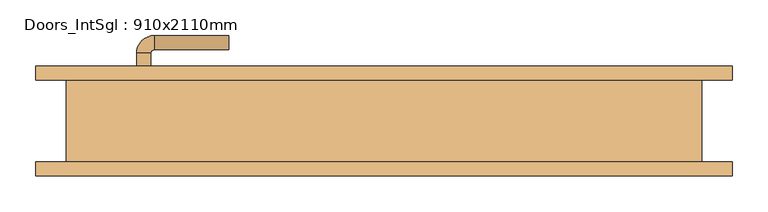
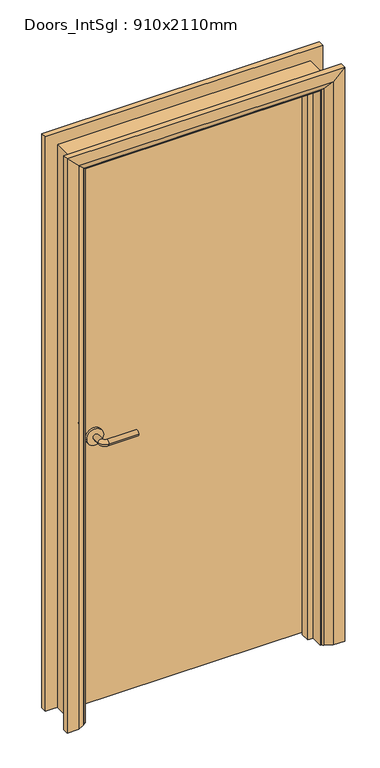
"""IFC4 building model written with IfcOpenShell, lengths in millimetres: door geometry, Doors_IntSgl : 910x2110mm."""

import ifcopenshell
import ifcopenshell.guid

model = None  # the IFC model being written
_history = None  # IfcOwnerHistory: only IFC2X3 demands one
_inside = {}  # id of a spatial element -> (the spatial element, [elements in it])
_under = {}  # id of a project, library or spatial element -> (it, [spatial elements below it])
_declared = {}  # id of a project -> (the project, [libraries it declares])
_typed = {}  # id of a type object -> (the type object, [elements of that type])
_made_of = {}  # id of a material, layer set ... -> (it, [elements and type objects made of it])


def new_model(schema):
    """Start an empty IFC model of exactly this schema.

    Asked for "IFC4X3", IfcOpenShell would pick the latest addendum, in which some entities
    have other attributes; the version numbers below select the first issue.
    IFC2X3 requires an IfcOwnerHistory on every rooted entity: one is made here for all.
    """
    global model, _history
    if schema == "IFC4X3":
        model = ifcopenshell.file(schema_version=(4, 3, 0, 0))
    else:
        model = ifcopenshell.file(schema=schema)
    _inside.clear()
    _under.clear()
    _declared.clear()
    _typed.clear()
    _made_of.clear()
    _history = None
    if model.schema == "IFC2X3":
        org = make("IfcOrganization", Name="unknown")
        user = make(
            "IfcPersonAndOrganization",
            ThePerson=make("IfcPerson", FamilyName="unknown"),
            TheOrganization=org,
        )
        app = make(
            "IfcApplication",
            ApplicationDeveloper=org,
            Version="unknown",
            ApplicationFullName="unknown",
            ApplicationIdentifier="unknown",
        )
        _history = make(
            "IfcOwnerHistory",
            OwningUser=user,
            OwningApplication=app,
            ChangeAction="ADDED",
            CreationDate=0,
        )
    return model


def make(cls, **values):
    """One entity of the class cls with the attributes given. An attribute that is None is left unset."""
    return model.create_entity(
        cls, **{name: value for name, value in values.items() if value is not None}
    )


def rooted(cls, **values):
    """An entity with a GlobalId (a new one), such as an element, a storey or a relation."""
    return make(cls, GlobalId=ifcopenshell.guid.new(), OwnerHistory=_history, **values)


def si_unit(unit_type, name, prefix=None):
    """IfcSIUnit, for example si_unit("LENGTHUNIT", "METRE", prefix="MILLI")."""
    return make("IfcSIUnit", UnitType=unit_type, Prefix=prefix, Name=name)


def assignment(units):
    """IfcUnitAssignment: the units of a project."""
    return None if units is None else make("IfcUnitAssignment", Units=units)


def point(xyz):
    """IfcCartesianPoint."""
    return None if xyz is None else make("IfcCartesianPoint", Coordinates=xyz)


def direction(xyz):
    """IfcDirection."""
    return None if xyz is None else make("IfcDirection", DirectionRatios=xyz)


def frame(location, z_axis=None, x_axis=None):
    """IfcAxis2Placement3D, a coordinate frame: its origin and axes. An axis left out is left unset."""
    return make(
        "IfcAxis2Placement3D",
        Location=point(location),
        Axis=direction(z_axis),
        RefDirection=direction(x_axis),
    )


def frame_2d(location, x_axis=None):
    """IfcAxis2Placement2D, a coordinate frame in the plane: its origin and x axis."""
    return make(
        "IfcAxis2Placement2D", Location=point(location), RefDirection=direction(x_axis)
    )


def origin():
    """The frame at (0, 0, 0) with its axes left unset."""
    return frame((0.0, 0.0, 0.0))


def place(relative_to, where):
    """IfcLocalPlacement: puts the frame where relative to a parent placement (None: the world)."""
    return make(
        "IfcLocalPlacement", PlacementRelTo=relative_to, RelativePlacement=where
    )


def context(
    kind, dimensions, precision=None, world=None, true_north=None, identifier=None
):
    """IfcGeometricRepresentationContext, for example the 3D "Model" context."""
    return make(
        "IfcGeometricRepresentationContext",
        ContextIdentifier=identifier,
        ContextType=kind,
        CoordinateSpaceDimension=dimensions,
        Precision=precision,
        WorldCoordinateSystem=world,
        TrueNorth=true_north,
    )


def project(units=None, contexts=None):
    """IfcProject with its units and contexts."""
    return rooted(
        "IfcProject",
        Name="project",
        RepresentationContexts=contexts,
        UnitsInContext=assignment(units),
    )


def spatial(cls, under=None, at=None, **own):
    """A site, building, storey or space (cls), placed at a placement, below another one or the project."""
    s = rooted(cls, ObjectPlacement=at, **own)
    if under is not None:
        _under.setdefault(under.id(), (under, []))[1].append(s)
    return s


def polyline(points):
    """IfcPolyline through the points."""
    return make("IfcPolyline", Points=[point(p) for p in points])


def circle_curve(where, radius):
    """IfcCircle in the frame where."""
    return make("IfcCircle", Position=where, Radius=radius)


def ellipse_curve(where, semi_axis1, semi_axis2):
    """IfcEllipse in the frame where."""
    return make(
        "IfcEllipse", Position=where, SemiAxis1=semi_axis1, SemiAxis2=semi_axis2
    )


def trimmed(basis, trim1, trim2, sense, master):
    """IfcTrimmedCurve: the piece of a basis curve between two trims."""
    return make(
        "IfcTrimmedCurve",
        BasisCurve=basis,
        Trim1=trim1,
        Trim2=trim2,
        SenseAgreement=sense,
        MasterRepresentation=master,
    )


def segment(curve, same_sense, transition):
    """IfcCompositeCurveSegment."""
    return make(
        "IfcCompositeCurveSegment",
        Transition=transition,
        SameSense=same_sense,
        ParentCurve=curve,
    )


def composite_curve(segments, self_intersect=None):
    """IfcCompositeCurve: segments joined end to end."""
    return make("IfcCompositeCurve", Segments=segments, SelfIntersect=self_intersect)


def outline(outer, holes=None, kind="AREA"):
    """IfcArbitraryClosedProfileDef: a profile drawn as a closed curve; with holes, ...WithVoids."""
    if holes is None:
        return make("IfcArbitraryClosedProfileDef", ProfileType=kind, OuterCurve=outer)
    return make(
        "IfcArbitraryProfileDefWithVoids",
        ProfileType=kind,
        OuterCurve=outer,
        InnerCurves=holes,
    )


def extrude(swept, where, along, depth):
    """IfcExtrudedAreaSolid: the profile swept, set in the frame where, extruded along a direction by depth."""
    return make(
        "IfcExtrudedAreaSolid",
        SweptArea=swept,
        Position=where,
        ExtrudedDirection=direction(along),
        Depth=depth,
    )


def faces_of(points, faces, orient=None, outer=None):
    """IfcFace entities. A face is a list of loops; a loop is a list of indices into points, from 0.

    orient and outer hold one flag for each loop. By default every Orientation is true, the
    first loop of a face is its IfcFaceOuterBound and the others are IfcFaceBound.
    """
    made = []
    for i, loops in enumerate(faces):
        bounds = []
        for j, loop in enumerate(loops):
            is_outer = j == 0 if outer is None else outer[i][j]
            bounds.append(
                make(
                    "IfcFaceOuterBound" if is_outer else "IfcFaceBound",
                    Bound=make("IfcPolyLoop", Polygon=[points[k] for k in loop]),
                    Orientation=True if orient is None else orient[i][j],
                )
            )
        made.append(make("IfcFace", Bounds=bounds))
    return made


def faceted_brep(points, faces, orient=None, outer=None, voids=None):
    """IfcFacetedBrep: a solid bounded by flat faces; with voids (closed shells), ...WithVoids."""
    shared = [point(p) for p in points]
    hull = make("IfcClosedShell", CfsFaces=faces_of(shared, faces, orient, outer))
    if voids is None:
        return make("IfcFacetedBrep", Outer=hull)
    return make(
        "IfcFacetedBrepWithVoids",
        Outer=hull,
        Voids=[
            make(cls, CfsFaces=faces_of(shared, fs, o, b)) for cls, fs, o, b in voids
        ],
    )


def shape(context_of_items, identifier, shape_type, items):
    """IfcShapeRepresentation: the items that make up one representation, for example the "Body"."""
    return make(
        "IfcShapeRepresentation",
        ContextOfItems=context_of_items,
        RepresentationIdentifier=identifier,
        RepresentationType=shape_type,
        Items=items,
    )


def source(mapping_origin, context_of_items, identifier, shape_type, items):
    """IfcRepresentationMap: a shape defined once, which mapped items show again and again."""
    return make(
        "IfcRepresentationMap",
        MappingOrigin=mapping_origin,
        MappedRepresentation=shape(context_of_items, identifier, shape_type, items),
    )


def transform(
    local_origin,
    x_axis=None,
    y_axis=None,
    z_axis=None,
    scale=None,
    scale2=None,
    scale3=None,
    uniform=True,
):
    """IfcCartesianTransformationOperator3D, or its non-uniform kind. x_axis, y_axis, z_axis: its Axis1, 2, 3."""
    if uniform:
        return make(
            "IfcCartesianTransformationOperator3D",
            Axis1=direction(x_axis),
            Axis2=direction(y_axis),
            LocalOrigin=point(local_origin),
            Scale=scale,
            Axis3=direction(z_axis),
        )
    return make(
        "IfcCartesianTransformationOperator3DnonUniform",
        Axis1=direction(x_axis),
        Axis2=direction(y_axis),
        LocalOrigin=point(local_origin),
        Scale=scale,
        Axis3=direction(z_axis),
        Scale2=scale2,
        Scale3=scale3,
    )


def mapped(mapping_source, mapping_target):
    """IfcMappedItem: shows the shape of a source again, moved by a transform."""
    return make(
        "IfcMappedItem", MappingSource=mapping_source, MappingTarget=mapping_target
    )


def made_of(thing, what):
    """Note that an element or type object is made of a material, layer set ...; save() writes the relation."""
    if what is not None:
        _made_of.setdefault(what.id(), (what, []))[1].append(thing)
    return thing


def element(
    cls,
    number,
    at=None,
    inside=None,
    cuts=None,
    type_object=None,
    material=None,
    context=None,
    identifier="Body",
    shape_type=None,
    held_by="IfcProductDefinitionShape",
    body=None,
    shapes=None,
    **own,
):
    """One element of the class cls, such as IfcWall. Its Tag is "e" and its number.

    at: its placement. inside: the storey or other place that contains it. cuts: it is an
    opening in that element (IfcRelVoidsElement). A single representation is given by context,
    identifier, shape_type and body (its items); several are given by shapes. held_by: the class
    of the entity that holds the representations. save() writes the other relations.
    """
    e = rooted(cls, Tag="e%d" % number, ObjectPlacement=at, **own)
    if body is not None:
        shapes = [shape(context, identifier, shape_type, body)]
    if shapes is not None:
        e.Representation = make(held_by, Representations=shapes)
    if inside is not None:
        _inside.setdefault(inside.id(), (inside, []))[1].append(e)
    if cuts is not None:
        rooted(
            "IfcRelVoidsElement", RelatingBuildingElement=cuts, RelatedOpeningElement=e
        )
    if type_object is not None:
        _typed.setdefault(type_object.id(), (type_object, []))[1].append(e)
    return made_of(e, material)


def aggregate(whole, parts):
    """IfcRelAggregates: a whole, such as a stair, and the parts it consists of."""
    return rooted("IfcRelAggregates", RelatingObject=whole, RelatedObjects=parts)


def save(model, path):
    """Write the relations noted so far, then the file.

    IfcRelAggregates (storeys below a building ...), IfcRelContainedInSpatialStructure (elements
    in a storey), IfcRelDefinesByType, IfcRelAssociatesMaterial and IfcRelDeclares: one each for
    every whole, place, type object, material and project.
    """
    for whole, parts in _under.values():
        aggregate(whole, parts)
    for where, things in _inside.values():
        rooted(
            "IfcRelContainedInSpatialStructure",
            RelatedElements=things,
            RelatingStructure=where,
        )
    for kind, things in _typed.values():
        rooted("IfcRelDefinesByType", RelatedObjects=things, RelatingType=kind)
    for what, things in _made_of.values():
        rooted("IfcRelAssociatesMaterial", RelatedObjects=things, RelatingMaterial=what)
    for by, libraries in _declared.values():
        rooted("IfcRelDeclares", RelatingContext=by, RelatedDefinitions=libraries)
    model.write(path)


def plane_surface(at):
    """IfcPlane: the flat surface through the origin of the frame at, square to its z axis."""
    return make("IfcPlane", Position=at)


def cylinder_surface(at, radius):
    """IfcCylindricalSurface: all points at the distance radius from the z axis of the frame at."""
    return make("IfcCylindricalSurface", Position=at, Radius=radius)


def revolved_surface(curve, axis_point, axis_direction):
    """IfcSurfaceOfRevolution: the curve turned about the line through axis_point along axis_direction."""
    return make(
        "IfcSurfaceOfRevolution",
        SweptCurve=make("IfcArbitraryOpenProfileDef", ProfileType="CURVE", Curve=curve),
        AxisPosition=make("IfcAxis1Placement", Location=point(axis_point), Axis=direction(axis_direction)),
    )


def advanced_brep(points, edges, surfaces, faces):
    """IfcAdvancedBrep: a solid bounded by faces that lie on surfaces and meet in shared edges.

    An edge is (start, end): straight between two places in points (the first is 0);
    or (start, end, curve); or (start, end, curve, False) where it runs against its curve.
    A face is (place in surfaces, loops), or (place, loops, False) where it looks against
    its surface's normal. A loop lists edges by number (the first is 1), with a minus sign
    where the edge is run from its end to its start. The first loop is the outer one.
    """
    corners = [point(p) for p in points]
    vertices = [make("IfcVertexPoint", VertexGeometry=c) for c in corners]
    made = []
    for start, end, *more in edges:
        made.append(
            make(
                "IfcEdgeCurve",
                EdgeStart=vertices[start],
                EdgeEnd=vertices[end],
                EdgeGeometry=more[0] if more else make("IfcPolyline", Points=[corners[start], corners[end]]),
                SameSense=more[1] if len(more) > 1 else True,
            )
        )
    hull = []
    for where, loops, *sense in faces:
        bounds = []
        for j, loop in enumerate(loops):
            ring = [make("IfcOrientedEdge", EdgeElement=made[abs(k) - 1], Orientation=k > 0) for k in loop]
            bounds.append(
                make(
                    "IfcFaceOuterBound" if j == 0 else "IfcFaceBound",
                    Bound=make("IfcEdgeLoop", EdgeList=ring),
                    Orientation=True,
                )
            )
        hull.append(make("IfcAdvancedFace", Bounds=bounds, FaceSurface=surfaces[where], SameSense=sense[0] if sense else True))
    return make("IfcAdvancedBrep", Outer=make("IfcClosedShell", CfsFaces=hull))


def doors_intsgl_910x2110mm_43063e6c(model_context):
    return source(origin(), model_context, "Body", "SolidModel", [
        advanced_brep(
        [(-348.0, 11.5, 1000.0), (-328.0, 11.5, 1000.0), (-328.0, -18.5, 1000.0), (-348.0, -18.5, 1000.0), (-323.0, -23.5, 1000.0), (-323.0, -43.5, 1000.0), (-218.0, -43.5, 1000.0), (-218.0, -23.5, 1000.0)],
        [
            (0, 1, circle_curve(frame((-338.0, 11.5, 1000.0), z_axis=(0.0, 1.0, 0.0), x_axis=(1.0, 0.0, 0.0)), 10.0)),
            (1, 0, circle_curve(frame((-338.0, 11.5, 1000.0), z_axis=(0.0, 1.0, 0.0), x_axis=(1.0, 0.0, 0.0)), 10.0)),
            (1, 2),
            (2, 3, circle_curve(frame((-338.0, -18.5, 1000.0), z_axis=(0.0, 1.0, 0.0), x_axis=(1.0, 0.0, 0.0)), 10.0)),
            (3, 0),
            (3, 2, circle_curve(frame((-338.0, -18.5, 1000.0), z_axis=(0.0, 1.0, 0.0), x_axis=(1.0, 0.0, 0.0)), 10.0)),
            (4, 5, circle_curve(frame((-323.0, -33.5, 1000.0), z_axis=(-1.0, 0.0, 0.0), x_axis=(0.0, 1.0, 0.0)), 10.0)),
            (5, 3, circle_curve(frame((-323.0, -18.5, 1000.0), z_axis=(0.0, 0.0, -1.0), x_axis=(-1.0, 0.0, 0.0)), 25.0)),
            (2, 4, circle_curve(frame((-323.0, -18.5, 1000.0), z_axis=(0.0, 0.0, 1.0), x_axis=(-1.0, 0.0, 0.0)), 5.0)),
            (5, 4, circle_curve(frame((-323.0, -33.5, 1000.0), z_axis=(-1.0, 0.0, 0.0), x_axis=(0.0, 1.0, 0.0)), 10.0)),
            (6, 7, circle_curve(frame((-218.0, -33.5, 1000.0), z_axis=(1.0, 0.0, 0.0), x_axis=(0.0, 1.0, 0.0)), 10.0)),
            (7, 6, circle_curve(frame((-218.0, -33.5, 1000.0), z_axis=(1.0, 0.0, 0.0), x_axis=(0.0, 1.0, 0.0)), 10.0)),
            (4, 7),
            (6, 5),
        ],
        [
            plane_surface(frame((-338.0, 11.5, 1000.0), z_axis=(0.0, 1.0, 0.0), x_axis=(0.0, 0.0, 1.0))),
            cylinder_surface(frame((-338.0, 11.5, 1000.0), z_axis=(0.0, 1.0, 0.0), x_axis=(1.0, 0.0, 0.0)), 10.0),
            revolved_surface(trimmed(ellipse_curve(frame((-338.0, -18.5, 1000.0), z_axis=(0.0, -1.0, 0.0), x_axis=(1.0, 0.0, 0.0)), 10.0, 10.0), [point((-348.0, -18.5, 1000.0))], [point((-328.0, -18.5, 1000.0))], True, "CARTESIAN"), (-323.0, -18.5, 1000.0), (0.0, 0.0, -1.0)),
            revolved_surface(trimmed(ellipse_curve(frame((-338.0, -18.5, 1000.0), z_axis=(0.0, -1.0, 0.0), x_axis=(1.0, 0.0, 0.0)), 10.0, 10.0), [point((-328.0, -18.5, 1000.0))], [point((-348.0, -18.5, 1000.0))], True, "CARTESIAN"), (-323.0, -18.5, 1000.0), (0.0, 0.0, -1.0)),
            plane_surface(frame((-218.0, -33.5, 1000.0), z_axis=(1.0, 0.0, 0.0), x_axis=(0.0, 0.0, 1.0))),
            cylinder_surface(frame((-323.0, -33.5, 1000.0), z_axis=(-1.0, 0.0, 0.0), x_axis=(0.0, 1.0, 0.0)), 10.0),
        ],
        [
            (0, [[1, 2]]),
            (1, [[3, 4, 5, -2]]),
            (1, [[-5, 6, -3, -1]]),
            (2, [[7, 8, -4, 9]]),
            (3, [[10, -9, -6, -8]]),
            (4, [[11, 12]]),
            (5, [[13, -11, 14, -7]]),
            (5, [[-14, -12, -13, -10]]),
        ],
    ),
        extrude(outline(composite_curve([segment(trimmed(circle_curve(frame_2d((1000.0, -340.5)), 30.0), [point((1000.0, -370.5))], [point((1000.0, -310.5))], False, "CARTESIAN"), True, "CONTINUOUS"), segment(trimmed(circle_curve(frame_2d((1000.0, -340.5)), 30.0), [point((1000.0, -310.5))], [point((1000.0, -370.5))], False, "CARTESIAN"), True, "CONTINUOUS")], self_intersect=False)), frame((0.0, 11.5, 0.0), z_axis=(0.0, 1.0, 0.0), x_axis=(0.0, 0.0, 1.0)), (0.0, 0.0, 1.0), 8.0),
        advanced_brep(
        [(-348.0, 65.5, 1000.0), (-328.0, 65.5, 1000.0), (-348.0, 95.5, 1000.0), (-328.0, 95.5, 1000.0), (-323.0, 100.5, 1000.0), (-323.0, 120.5, 1000.0), (-218.0, 120.5, 1000.0), (-218.0, 100.5, 1000.0)],
        [
            (0, 1, circle_curve(frame((-338.0, 65.5, 1000.0), z_axis=(0.0, -1.0, 0.0), x_axis=(1.0, 0.0, 0.0)), 10.0)),
            (1, 0, circle_curve(frame((-338.0, 65.5, 1000.0), z_axis=(0.0, -1.0, 0.0), x_axis=(1.0, 0.0, 0.0)), 10.0)),
            (0, 2),
            (2, 3, circle_curve(frame((-338.0, 95.5, 1000.0), z_axis=(0.0, -1.0, 0.0), x_axis=(1.0, 0.0, 0.0)), 10.0)),
            (3, 1),
            (3, 2, circle_curve(frame((-338.0, 95.5, 1000.0), z_axis=(0.0, -1.0, 0.0), x_axis=(1.0, 0.0, 0.0)), 10.0)),
            (4, 3, circle_curve(frame((-323.0, 95.5, 1000.0), z_axis=(0.0, 0.0, 1.0), x_axis=(-1.0, 0.0, 0.0)), 5.0)),
            (2, 5, circle_curve(frame((-323.0, 95.5, 1000.0), z_axis=(0.0, 0.0, -1.0), x_axis=(-1.0, 0.0, 0.0)), 25.0)),
            (5, 4, circle_curve(frame((-323.0, 110.5, 1000.0), z_axis=(-1.0, 0.0, 0.0), x_axis=(0.0, -1.0, 0.0)), 10.0)),
            (4, 5, circle_curve(frame((-323.0, 110.5, 1000.0), z_axis=(-1.0, 0.0, 0.0), x_axis=(0.0, -1.0, 0.0)), 10.0)),
            (6, 7, circle_curve(frame((-218.0, 110.5, 1000.0), z_axis=(1.0, 0.0, 0.0), x_axis=(0.0, -1.0, 0.0)), 10.0)),
            (7, 6, circle_curve(frame((-218.0, 110.5, 1000.0), z_axis=(1.0, 0.0, 0.0), x_axis=(0.0, -1.0, 0.0)), 10.0)),
            (5, 6),
            (7, 4),
        ],
        [
            plane_surface(frame((-338.0, 65.5, 1000.0), z_axis=(0.0, -1.0, 0.0), x_axis=(0.0, 0.0, 1.0))),
            cylinder_surface(frame((-338.0, 65.5, 1000.0), z_axis=(0.0, -1.0, 0.0), x_axis=(1.0, 0.0, 0.0)), 10.0),
            revolved_surface(trimmed(ellipse_curve(frame((-338.0, 95.5, 1000.0), z_axis=(0.0, -1.0, 0.0), x_axis=(1.0, 0.0, 0.0)), 10.0, 10.0), [point((-348.0, 95.5, 1000.0))], [point((-328.0, 95.5, 1000.0))], True, "CARTESIAN"), (-323.0, 95.5, 1000.0), (0.0, 0.0, -1.0)),
            revolved_surface(trimmed(ellipse_curve(frame((-338.0, 95.5, 1000.0), z_axis=(0.0, -1.0, 0.0), x_axis=(1.0, 0.0, 0.0)), 10.0, 10.0), [point((-328.0, 95.5, 1000.0))], [point((-348.0, 95.5, 1000.0))], True, "CARTESIAN"), (-323.0, 95.5, 1000.0), (0.0, 0.0, -1.0)),
            plane_surface(frame((-218.0, 110.5, 1000.0), z_axis=(1.0, 0.0, 0.0), x_axis=(0.0, 0.0, 1.0))),
            cylinder_surface(frame((-323.0, 110.5, 1000.0), z_axis=(-1.0, 0.0, 0.0), x_axis=(0.0, -1.0, 0.0)), 10.0),
        ],
        [
            (0, [[1, 2]]),
            (1, [[-1, 3, 4, 5]]),
            (1, [[-2, -5, 6, -3]]),
            (2, [[7, -4, 8, 9]]),
            (3, [[-8, -6, -7, 10]]),
            (4, [[11, 12]]),
            (5, [[-9, 13, -12, 14]]),
            (5, [[-10, -14, -11, -13]]),
        ],
    ),
        extrude(outline(composite_curve([segment(trimmed(circle_curve(frame_2d((1000.0, -340.5)), 30.0), [point((1000.0, -370.5))], [point((1000.0, -310.5))], False, "CARTESIAN"), True, "CONTINUOUS"), segment(trimmed(circle_curve(frame_2d((1000.0, -340.5)), 30.0), [point((1000.0, -310.5))], [point((1000.0, -370.5))], False, "CARTESIAN"), True, "CONTINUOUS")], self_intersect=False)), frame((0.0, 57.5, 0.0), z_axis=(0.0, 1.0, 0.0), x_axis=(0.0, 0.0, 1.0)), (0.0, 0.0, 1.0), 8.0),
        extrude(outline(polyline([(413.0, 19.5), (-413.0, 19.5), (-413.0, 57.5), (413.0, 57.5), (413.0, 19.5)])), frame((0.0, 0.0, 8.0), z_axis=(0.0, 0.0, 1.0), x_axis=(1.0, 0.0, 0.0)), (0.0, 0.0, 1.0), 2060.0),
        advanced_brep(
        [(490.0, 77.5, 0.0), (490.0, 57.5, 0.0), (420.0, 57.5, 0.0), (424.0, 63.5, 0.0), (450.0, 77.5, 0.0), (490.0, 77.5, 2145.0), (490.0, 57.5, 2145.0), (-490.0, 57.5, 2145.0), (-490.0, 57.5, 0.0), (-420.0, 57.5, 0.0), (-420.0, 57.5, 2075.0), (420.0, 57.5, 2075.0), (424.0, 63.5, 2079.0), (450.0, 77.5, 2105.0), (-450.0, 77.5, 2105.0), (-450.0, 77.5, 0.0), (-490.0, 77.5, 0.0), (-490.0, 77.5, 2145.0), (-424.0, 63.5, 2079.0), (-424.0, 63.5, 0.0)],
        [
            (0, 1),
            (1, 2),
            (2, 3, circle_curve(frame((428.0, 56.5, 0.0), z_axis=(0.0, 0.0, -1.0), x_axis=(1.0, 0.0, 0.0)), 8.0622577)),
            (3, 4),
            (4, 0),
            (0, 5),
            (5, 6),
            (6, 1),
            (6, 7),
            (7, 8),
            (8, 9),
            (9, 10),
            (10, 11),
            (11, 2),
            (11, 12, ellipse_curve(frame((428.0, 56.5, 2083.0), z_axis=(0.7071067811865475, 0.0, -0.7071067811865475), x_axis=(-0.7071067811865474, 0.0, -0.7071067811865476)), 11.4017543, 8.0622577)),
            (12, 3),
            (12, 13),
            (13, 4),
            (13, 14),
            (14, 15),
            (15, 16),
            (16, 17),
            (17, 5),
            (17, 7),
            (10, 18, ellipse_curve(frame((-428.0, 56.5, 2083.0), z_axis=(0.7071067811865475, 0.0, 0.7071067811865475), x_axis=(0.7071067811865476, 0.0, -0.7071067811865474)), 11.4017543, 8.0622577)),
            (18, 12),
            (18, 14),
            (15, 19),
            (19, 9, circle_curve(frame((-428.0, 56.5, 0.0), z_axis=(0.0, 0.0, -1.0), x_axis=(-1.0, 0.0, 0.0)), 8.0622577)),
            (8, 16),
            (19, 18),
        ],
        [
            plane_surface(frame((420.0, 57.5, 0.0), z_axis=(0.0, 0.0, -1.0), x_axis=(0.0, -1.0, 0.0))),
            plane_surface(frame((490.0, 77.5, 0.0), z_axis=(1.0, 0.0, 0.0), x_axis=(0.0, 0.0, 1.0))),
            plane_surface(frame((490.0, 57.5, 0.0), z_axis=(0.0, -1.0, 0.0), x_axis=(0.0, 0.0, 1.0))),
            cylinder_surface(frame((428.0, 56.5, 0.0), z_axis=(0.0, 0.0, -1.0), x_axis=(1.0, 0.0, 0.0)), 8.0622577),
            plane_surface(frame((424.0, 63.5, 0.0), z_axis=(-0.4740998230350126, 0.880471099922178, 0.0), x_axis=(0.0, 0.0, 1.0))),
            plane_surface(frame((450.0, 77.5, 0.0), z_axis=(0.0, 1.0, 0.0), x_axis=(0.0, 0.0, 1.0))),
            plane_surface(frame((490.0, 77.5, 2145.0), z_axis=(0.0, 0.0, 1.0), x_axis=(-1.0, 0.0, 0.0))),
            cylinder_surface(frame((420.0, 56.5, 2083.0), z_axis=(1.0, 0.0, 0.0), x_axis=(0.0, 0.0, 1.0)), 8.0622577),
            plane_surface(frame((424.0, 63.5, 2079.0), z_axis=(0.0, 0.8804710999221764, -0.4740998230350154), x_axis=(-1.0, 0.0, 0.0))),
            plane_surface(frame((-420.0, 57.5, 0.0), z_axis=(0.0, 0.0, -1.0), x_axis=(0.0, -1.0, 0.0))),
            plane_surface(frame((-490.0, 77.5, 2145.0), z_axis=(-1.0, 0.0, 0.0), x_axis=(0.0, 0.0, -1.0))),
            cylinder_surface(frame((-428.0, 56.5, 2075.0), z_axis=(0.0, 0.0, 1.0), x_axis=(-1.0, 0.0, 0.0)), 8.0622577),
            plane_surface(frame((-424.0, 63.5, 2079.0), z_axis=(0.47409982303501824, 0.8804710999221749, 0.0), x_axis=(0.0, 0.0, -1.0))),
        ],
        [
            (0, [[1, 2, 3, 4, 5]]),
            (1, [[-1, 6, 7, 8]]),
            (2, [[-2, -8, 9, 10, 11, 12, 13, 14]]),
            (3, [[-3, -14, 15, 16]]),
            (4, [[-4, -16, 17, 18]]),
            (5, [[-5, -18, 19, 20, 21, 22, 23, -6]]),
            (6, [[-7, -23, 24, -9]]),
            (7, [[-15, -13, 25, 26]]),
            (8, [[-17, -26, 27, -19]]),
            (9, [[-21, 28, 29, -11, 30]]),
            (10, [[-24, -22, -30, -10]]),
            (11, [[-25, -12, -29, 31]]),
            (12, [[-27, -31, -28, -20]]),
        ],
    ),
        extrude(outline(polyline([(0.0, -415.0), (0.0, -396.0), (2051.0, -396.0), (2051.0, 396.0), (0.0, 396.0), (0.0, 415.0), (2070.0, 415.0), (2070.0, -415.0), (0.0, -415.0)])), frame((0.0, -14.5, 0.0), z_axis=(0.0, 1.0, 0.0), x_axis=(0.0, 0.0, 1.0)), (0.0, 0.0, 1.0), 32.0),
        advanced_brep(
        [(-490.0, -77.5, 0.0), (-490.0, -57.5, 0.0), (-420.0, -57.5, 0.0), (-424.0, -63.5, 0.0), (-450.0, -77.5, 0.0), (-490.0, -77.5, 2145.0), (-490.0, -57.5, 2145.0), (-420.0, -57.5, 2075.0), (-424.0, -63.5, 2079.0), (-450.0, -77.5, 2105.0), (490.0, -77.5, 2145.0), (490.0, -57.5, 2145.0), (420.0, -57.5, 2075.0), (424.0, -63.5, 2079.0), (450.0, -77.5, 2105.0), (490.0, -77.5, 0.0), (450.0, -77.5, 0.0), (424.0, -63.5, 0.0), (420.0, -57.5, 0.0), (490.0, -57.5, 0.0)],
        [
            (0, 1),
            (1, 2),
            (2, 3, circle_curve(frame((-428.0, -56.5, 0.0), z_axis=(0.0, 0.0, -1.0), x_axis=(-1.0, 0.0, 0.0)), 8.0622577)),
            (3, 4),
            (4, 0),
            (0, 5),
            (5, 6),
            (6, 1),
            (6, 7),
            (7, 2),
            (7, 8, ellipse_curve(frame((-428.0, -56.5, 2083.0), z_axis=(-0.7071067811865475, 0.0, -0.7071067811865475), x_axis=(0.7071067811865474, 0.0, -0.7071067811865476)), 11.4017543, 8.0622577)),
            (8, 3),
            (8, 9),
            (9, 4),
            (9, 5),
            (5, 10),
            (10, 11),
            (11, 6),
            (11, 12),
            (12, 7),
            (12, 13, ellipse_curve(frame((428.0, -56.5, 2083.0), z_axis=(-0.7071067811865475, 0.0, 0.7071067811865475), x_axis=(-0.7071067811865476, 0.0, -0.7071067811865474)), 11.4017543, 8.0622577)),
            (13, 8),
            (13, 14),
            (14, 9),
            (14, 10),
            (15, 16),
            (16, 17),
            (17, 18, circle_curve(frame((428.0, -56.5, 0.0), z_axis=(0.0, 0.0, -1.0), x_axis=(1.0, 0.0, 0.0)), 8.0622577)),
            (18, 19),
            (19, 15),
            (10, 15),
            (19, 11),
            (18, 12),
            (17, 13),
            (16, 14),
        ],
        [
            plane_surface(frame((-420.0, -130.3010989, 0.0), z_axis=(0.0, 0.0, -1.0), x_axis=(1.0, 0.0, 0.0))),
            plane_surface(frame((-490.0, -77.5, 0.0), z_axis=(-1.0, 0.0, 0.0), x_axis=(0.0, 0.0, 1.0))),
            plane_surface(frame((-490.0, -57.5, 0.0), z_axis=(0.0, 1.0, 0.0), x_axis=(0.0, 0.0, 1.0))),
            cylinder_surface(frame((-428.0, -56.5, 0.0), z_axis=(0.0, 0.0, -1.0), x_axis=(-1.0, 0.0, 0.0)), 8.0622577),
            plane_surface(frame((-424.0, -63.5, 0.0), z_axis=(0.4740998230350183, -0.8804710999221749, 0.0), x_axis=(0.0, 0.0, 1.0))),
            plane_surface(frame((-450.0, -77.5, 0.0), z_axis=(0.0, -1.0, 0.0), x_axis=(0.0, 0.0, 1.0))),
            plane_surface(frame((-490.0, -77.5, 2145.0), z_axis=(0.0, 0.0, 1.0), x_axis=(1.0, 0.0, 0.0))),
            plane_surface(frame((-490.0, -57.5, 2145.0), z_axis=(0.0, 1.0, 0.0), x_axis=(1.0, 0.0, 0.0))),
            cylinder_surface(frame((-420.0, -56.5, 2083.0), z_axis=(-1.0, 0.0, 0.0), x_axis=(0.0, 0.0, 1.0)), 8.0622577),
            plane_surface(frame((-424.0, -63.5, 2079.0), z_axis=(0.0, -0.8804710999221749, -0.4740998230350183), x_axis=(1.0, 0.0, 0.0))),
            plane_surface(frame((-450.0, -77.5, 2105.0), z_axis=(0.0, -1.0, 0.0), x_axis=(1.0, 0.0, 0.0))),
            plane_surface(frame((420.0, -130.3010989, 0.0), z_axis=(0.0, 0.0, -1.0), x_axis=(-1.0, 0.0, 0.0))),
            plane_surface(frame((490.0, -77.5, 2145.0), z_axis=(1.0, 0.0, 0.0), x_axis=(0.0, 0.0, -1.0))),
            plane_surface(frame((490.0, -57.5, 2145.0), z_axis=(0.0, 1.0, 0.0), x_axis=(0.0, 0.0, -1.0))),
            cylinder_surface(frame((428.0, -56.5, 2075.0), z_axis=(0.0, 0.0, 1.0), x_axis=(1.0, 0.0, 0.0)), 8.0622577),
            plane_surface(frame((424.0, -63.5, 2079.0), z_axis=(-0.4740998230350183, -0.8804710999221749, 0.0), x_axis=(0.0, 0.0, -1.0))),
            plane_surface(frame((450.0, -77.5, 2105.0), z_axis=(0.0, -1.0, 0.0), x_axis=(0.0, 0.0, -1.0))),
        ],
        [
            (0, [[1, 2, 3, 4, 5]]),
            (1, [[-1, 6, 7, 8]]),
            (2, [[-2, -8, 9, 10]]),
            (3, [[-3, -10, 11, 12]]),
            (4, [[-4, -12, 13, 14]]),
            (5, [[-5, -14, 15, -6]]),
            (6, [[-7, 16, 17, 18]]),
            (7, [[-9, -18, 19, 20]]),
            (8, [[-11, -20, 21, 22]]),
            (9, [[-13, -22, 23, 24]]),
            (10, [[-15, -24, 25, -16]]),
            (11, [[26, 27, 28, 29, 30]]),
            (12, [[-17, 31, -30, 32]]),
            (13, [[-19, -32, -29, 33]]),
            (14, [[-21, -33, -28, 34]]),
            (15, [[-23, -34, -27, 35]]),
            (16, [[-25, -35, -26, -31]]),
        ],
    ),
        faceted_brep([(-415.0, 57.5, 0.0), (-415.0, -57.5, 0.0), (-447.0, -57.5, 0.0), (-447.0, 57.5, 0.0), (-415.0, 57.5, 2070.0), (-415.0, -57.5, 2070.0), (-447.0, -57.5, 2102.0), (-447.0, 57.5, 2102.0), (415.0, 57.5, 2070.0), (415.0, -57.5, 2070.0), (447.0, -57.5, 2102.0), (447.0, 57.5, 2102.0), (415.0, 57.5, 0.0), (447.0, 57.5, 0.0), (447.0, -57.5, 0.0), (415.0, -57.5, 0.0)], [[[0, 1, 2, 3]], [[1, 0, 4, 5]], [[2, 1, 5, 6]], [[3, 2, 6, 7]], [[0, 3, 7, 4]], [[5, 4, 8, 9]], [[6, 5, 9, 10]], [[7, 6, 10, 11]], [[4, 7, 11, 8]], [[12, 13, 14, 15]], [[9, 8, 12, 15]], [[10, 9, 15, 14]], [[11, 10, 14, 13]], [[8, 11, 13, 12]]]),
    ])


if __name__ == "__main__":
    model = new_model("IFC4")
    model_context = context("Model", 3, world=origin())
    ifc_project = project(units=[si_unit("LENGTHUNIT", "METRE", prefix="MILLI")], contexts=[model_context])
    site = spatial("IfcSite", under=ifc_project)
    building = spatial("IfcBuilding", under=site)
    placement = place(None, origin())
    doors_intsgl_910x2110mm_shape = doors_intsgl_910x2110mm_43063e6c(model_context)
    element("IfcDoor", 1, ObjectType="Doors_IntSgl : 910x2110mm", at=placement, inside=building, context=model_context, shape_type="MappedRepresentation", body=[
        mapped(doors_intsgl_910x2110mm_shape, transform((0.0, 0.0, 0.0), x_axis=(1.0, 0.0, 0.0), y_axis=(0.0, 1.0, 0.0), z_axis=(0.0, 0.0, 1.0))),
    ])
    save(model, "model.ifc")

# Revit data of these elements
# Type "Doors_IntSgl : 910x2110mm"
#   Construction Type Id = "MDOOR"
#   Type Mark = "41"
#   Type Comments = "Internal Single"
#   Operation = "SingleSwingRight"
#   Manufacturer = "Revit"
#   Keynote = "L20"
#   Description = "Internal Single Door"
#   Analytic Construction = "Metal"
#   UnderCut = 8 mm
#   Tolerance = 2 mm
#   Thickness = 38 mm
#   Thermal Resistance (R) = 0.270117 (m²·K)/W
#   Structural Tolerance = 8 mm
#   StopDepth = 32 mm
#   Stop Thickness = 19 mm
#   Rough Width = 910 mm
#   Rough Height = 2110 mm
#   Height to Top Lock Rail = 1000 mm
#   Heat Transfer Coefficient (U) = 3.7021 W/(m²·K)
#   Handle Z Distance = 1000 mm
#   Handle X Distance = 75 mm
#   Frame Thickness = 32 mm
#   Door Panel Width = 826 mm
#   Door Panel Thickness = 38 mm
#   Door Panel Offset = 0 mm
#   Height = 2110 mm
#   Width = 910 mm
#   Door Panel Height = 2060 mm
#   Architrave Setback = 5 mm
#   Define Thermal Properties by = 1
#   Vis - Ironmongery = yes
#   Material Ironmongery = Door - Handle
#   Material Frame = Door - Frame/Mullion (1)
#   Material Door = Door - Panel
#   Material Architrave = Door - Architrave
#   Visual Light Transmittance = 0
#   Solar Heat Gain Coefficient = 0
#   Function = (empty or 0)
#   Wall Closure = (empty or 0)
# Element 1 (IfcDoor, "Doors_IntSgl : 910x2110mm")
#   Materials on its faces: "Door - Architrave", "Door - Handle", "Door - Frame/Mullion (1)", "Door - Panel"
# Materials
#   "Door - Handle": class "Miscellaneous", colour RGB 0 0 0, transparency 0, Keynote = "P21", Cost = 0
#   "Door - Frame/Mullion (1)": class "Wood", colour RGB 212 179 113, transparency 0, Keynote = "L20", Cost = 0
#   "Door - Panel": class "Wood", colour RGB 210 159 95, transparency 0, Keynote = "L20", Cost = 0
#   "Door - Architrave": class "Wood", colour RGB 154 90 5, transparency 0, Keynote = "P20", Cost = 0
